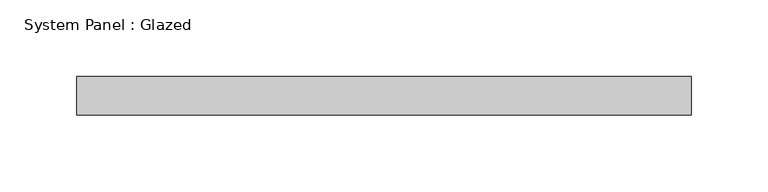
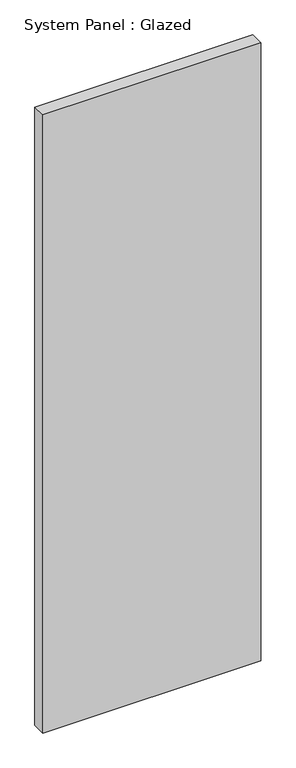
"""IFC4 building model written with IfcOpenShell, lengths in millimetres: plate geometry, System Panel : Glazed."""

from ifc_helpers import new_model, si_unit, origin, origin_with_axes, place, context, project, spatial, polyline, outline, extrude, source, transform, mapped, element, save


def system_panel_glazed_3e660766(model_context):
    return source(origin(), model_context, "Body", "SweptSolid", [
        extrude(outline(polyline([(200.0, 24.5), (-200.0, 24.5), (-200.0, 49.5), (200.0, 49.5), (200.0, 24.5)])), origin_with_axes(), (0.0, 0.0, 1.0), 1200.0),
    ])


if __name__ == "__main__":
    model = new_model("IFC4")
    model_context = context("Model", 3, world=origin())
    ifc_project = project(units=[si_unit("LENGTHUNIT", "METRE", prefix="MILLI")], contexts=[model_context])
    site = spatial("IfcSite", under=ifc_project)
    building = spatial("IfcBuilding", under=site)
    placement = place(None, origin())
    system_panel_glazed_shape = system_panel_glazed_3e660766(model_context)
    element("IfcPlate", 1, ObjectType="System Panel : Glazed", at=placement, inside=building, context=model_context, shape_type="MappedRepresentation", body=[
        mapped(system_panel_glazed_shape, transform((0.0, 0.0, 0.0), x_axis=(1.0, 0.0, 0.0), y_axis=(0.0, 1.0, 0.0), z_axis=(0.0, 0.0, 1.0))),
    ])
    save(model, "model.ifc")

# Revit data of these elements
# Element 1 (IfcPlate, "System Panel : Glazed")
#   Materials on its faces: "Glass"
# Materials
#   "Glass": class "Glass", colour RGB 218 227 224, transparency 0.85, Description = "Soda Lime Glass", Cost = 0
